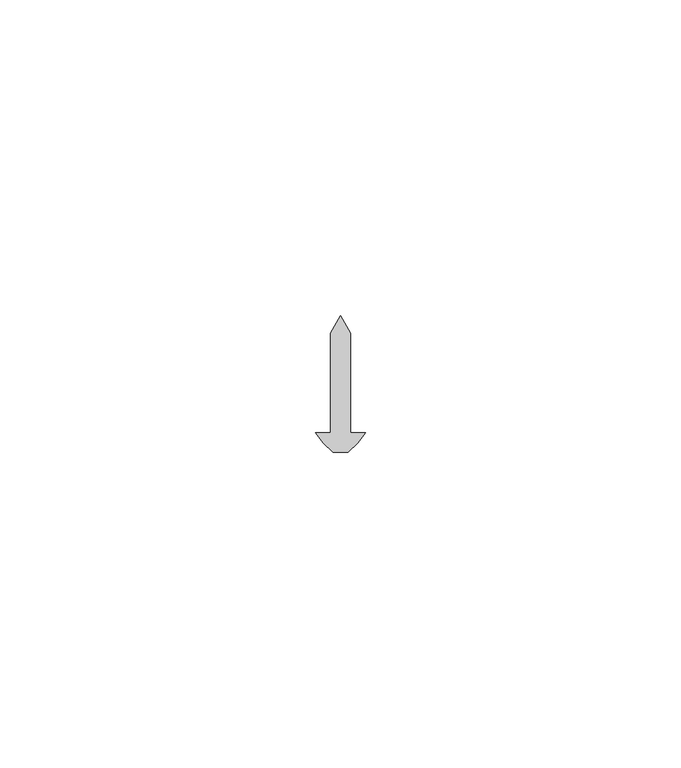
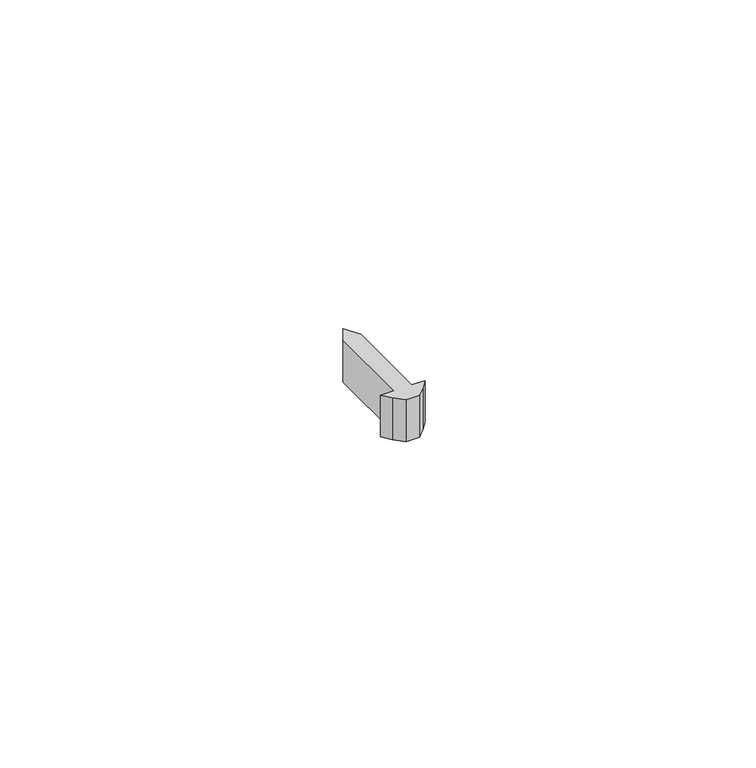
"""IFC4 building model written with IfcOpenShell, lengths in millimetres: proxy geometry, Generic Models 7:Generic Models 1:3:Generic Models 1:3 : Generic Models 7:Generic Models 1:305549:3:Generic Models 1:3:Generic Models 1:3 : Generic Models 7:Generic Models 1:305549:3 : Generic Models 7:Generic Models 1:3:Generic Models 1:3 : Generic Models 7:Generic Models 1:305549:301244:13 : Generic Models 7:Generic Models 1:3:Generic Models 1:3 : Generic Models 7:Generic Models 1:305549:3:Generic Models 1:3:Generic Models 1:3 : Generic Models 7:Generic Models 1:305549:3 : Generic Models 7:Generic Models 1:3:Generic Models 1:3 : Generic Models 7:Generic Models 1:305549:301244:308848."""

from ifc_helpers import new_model, si_unit, frame, origin, place, context, project, spatial, polyline, outline, extrude, source, transform, mapped, element, save


def generic_models_c6b2e827(model_context):
    return source(origin(), model_context, "Body", "SweptSolid", [
        extrude(outline(polyline([(579306.1242239, -579084.8288841), (579306.1242239, -579069.0196286), (579307.7117239, -579066.2699979), (579309.2992239, -579069.0196286), (579309.2992239, -579084.8288841), (579311.6804739, -579084.8288841), (579310.4622784, -579086.3559421), (579308.9103882, -579087.9078323), (579306.5130597, -579087.9078323), (579304.9611695, -579086.3559421), (579303.7429739, -579084.8288841), (579306.1242239, -579084.8288841)])), frame((0.0, 0.0, 4907.75625), z_axis=(0.0, 0.0, 1.0), x_axis=(1.0, 0.0, 0.0)), (0.0, 0.0, 1.0), 7.9375),
    ])


if __name__ == "__main__":
    model = new_model("IFC4")
    model_context = context("Model", 3, world=origin())
    ifc_project = project(units=[si_unit("LENGTHUNIT", "METRE", prefix="MILLI")], contexts=[model_context])
    site = spatial("IfcSite", under=ifc_project)
    building = spatial("IfcBuilding", under=site)
    placement = place(None, origin())
    generic_models_shape = generic_models_c6b2e827(model_context)
    element("IfcBuildingElementProxy", 1, Name="Generic Models 7:Generic Models 1:3:Generic Models 1:3 : Generic Models 7:Generic Models 1:305549:3:Generic Models 1:3:Generic Models 1:3 : Generic Models 7:Generic Models 1:305549:3 : Generic Models 7:Generic Models 1:3:Generic Models 1:3 : Generic Models 7:Generic Models 1:305549:301244:13 : Generic Models 7:Generic Models 1:3:Generic Models 1:3 : Generic Models 7:Generic Models 1:305549:3:Generic Models 1:3:Generic Models 1:3 : Generic Models 7:Generic Models 1:305549:3 : Generic Models 7:Generic Models 1:3:Generic Models 1:3 : Generic Models 7:Generic Models 1:305549:301244:308848", ObjectType="Generic Models 7:Generic Models 1:3:Generic Models 1:3 : Generic Models 7:Generic Models 1:305549:3:Generic Models 1:3:Generic Models 1:3 : Generic Models 7:Generic Models 1:305549:3 : Generic Models 7:Generic Models 1:3:Generic Models 1:3 : Generic Models 7:Generic Models 1:305549:301244:13 : Generic Models 7:Generic Models 1:3:Generic Models 1:3 : Generic Models 7:Generic Models 1:305549:3:Generic Models 1:3:Generic Models 1:3 : Generic Models 7:Generic Models 1:305549:3 : Generic Models 7:Generic Models 1:3:Generic Models 1:3 : Generic Models 7:Generic Models 1:305549:301244:308848", at=placement, inside=building, context=model_context, shape_type="MappedRepresentation", body=[
        mapped(generic_models_shape, transform((0.0, 0.0, 0.0), x_axis=(1.0, 0.0, 0.0), y_axis=(0.0, 1.0, 0.0), z_axis=(0.0, 0.0, 1.0))),
    ])
    save(model, "model.ifc")

# Revit data of these elements
# Type "Generic Models 7:Generic Models 1:3:Generic Models 1:3 : Generic Models 7:Generic Models 1:305549:3:Generic Models 1:3:Generic Models 1:3 : Generic Models 7:Generic Models 1:305549:3 : Generic Models 7:Generic Models 1:3:Generic Models 1:3 : Generic Models 7:Generic Models 1:305549:301244:13 : Generic Models 7:Generic Models 1:3:Generic Models 1:3 : Generic Models 7:Generic Models 1:305549:3:Generic Models 1:3:Generic Models 1:3 : Generic Models 7:Generic Models 1:305549:3 : Generic Models 7:Generic Models 1:3:Generic Models 1:3 : Generic Models 7:Generic Models 1:305549:301244:308848"
#   NameOverride = "Generic Models 7:Generic Models 1:3:Generic Models 1:3 : Generic Models 7:Generic Models 1:305549:3:Generic Models 1:3:Generic Models 1:3 : Generic Models 7:Generic Models 1:305549:3 : Generic Models 7:Generic Models 1:3:Generic Models 1:3 : Generic Models 7:Generic Models 1:305549:301244:308848"
#   ObjectTypeOverride = "Generic Models 1:3:Generic Models 1:3 : Generic Models 7:Generic Models 1:305549:3 : Generic Models 7:Generic Models 1:3:Generic Models 1:3 : Generic Models 7:Generic Models 1:305549:301244"
#   Reference = "Generic Models 1"
#   Tag = "308848"
# Element 1 (IfcBuildingElementProxy, "Generic Models 7:Generic Models 1:3:Generic Models 1:3 : Generic Models 7:Generic Models 1:305549:3:Generic Models 1:3:Generic Models 1:3 : Generic Models 7:Generic Models 1:305549:3 : Generic Models 7:Generic Models 1:3:Generic Models 1:3 : Generic Models 7:Generic Models 1:305549:301244:13 : Generic Models 7:Generic Models 1:3:Generic Models 1:3 : Generic Models 7:Generic Models 1:305549:3:Generic Models 1:3:Generic Models 1:3 : Generic Models 7:Generic Models 1:305549:3 : Generic Models 7:Generic Models 1:3:Generic Models 1:3 : Generic Models 7:Generic Models 1:305549:301244:308848")
#   Materials on its faces: "FASTENERS (T.B.D)"
# Materials
#   "FASTENERS (T.B.D)": class "Generic", colour RGB 120 120 120, transparency 0, Cost = 0
